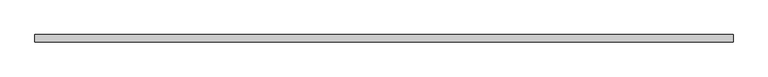
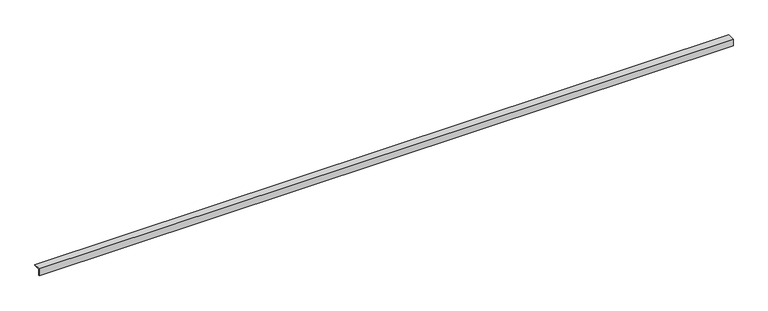
"""IFC4 building model written with IfcOpenShell, lengths in millimetres: proxy geometry, Generic Models 7:Generic Models 1:337419:Generic Models 1:337419 : Generic Models 7:Generic Models 1:337419:15 : Generic Models 7:Generic Models 1:337419:Generic Models 1:337419 : Generic Models 7:Generic Models 1:337419:301336."""

from ifc_helpers import new_model, si_unit, frame, origin, place, context, project, spatial, polyline, outline, extrude, source, transform, mapped, element, save


def generic_models_9543ae2d(model_context):
    return source(origin(), model_context, "Body", "SweptSolid", [
        extrude(outline(polyline([(-536554.1163358, 8576.3695313), (-536503.3163358, 8576.3695313), (-536503.3163358, 8571.6070313), (-536549.3538358, 8571.6070313), (-536549.3538358, 8525.5695312), (-536554.1163358, 8525.5695312), (-536554.1163358, 8576.3695313)])), frame((591306.0367242, 0.0, 0.0), z_axis=(1.0, 0.0, 0.0), x_axis=(0.0, 1.0, 0.0)), (0.0, 0.0, 1.0), 4876.8),
    ])


if __name__ == "__main__":
    model = new_model("IFC4")
    model_context = context("Model", 3, world=origin())
    ifc_project = project(units=[si_unit("LENGTHUNIT", "METRE", prefix="MILLI")], contexts=[model_context])
    site = spatial("IfcSite", under=ifc_project)
    building = spatial("IfcBuilding", under=site)
    placement = place(None, origin())
    generic_models_shape = generic_models_9543ae2d(model_context)
    element("IfcBuildingElementProxy", 1, Name="Generic Models 7:Generic Models 1:337419:Generic Models 1:337419 : Generic Models 7:Generic Models 1:337419:15 : Generic Models 7:Generic Models 1:337419:Generic Models 1:337419 : Generic Models 7:Generic Models 1:337419:301336", ObjectType="Generic Models 7:Generic Models 1:337419:Generic Models 1:337419 : Generic Models 7:Generic Models 1:337419:15 : Generic Models 7:Generic Models 1:337419:Generic Models 1:337419 : Generic Models 7:Generic Models 1:337419:301336", at=placement, inside=building, context=model_context, shape_type="MappedRepresentation", body=[
        mapped(generic_models_shape, transform((0.0, 0.0, 0.0), x_axis=(1.0, 0.0, 0.0), y_axis=(0.0, 1.0, 0.0), z_axis=(0.0, 0.0, 1.0))),
    ])
    save(model, "model.ifc")

# Revit data of these elements
# Type "Generic Models 7:Generic Models 1:337419:Generic Models 1:337419 : Generic Models 7:Generic Models 1:337419:15 : Generic Models 7:Generic Models 1:337419:Generic Models 1:337419 : Generic Models 7:Generic Models 1:337419:301336"
#   NameOverride = "Generic Models 7:Generic Models 1:337419:Generic Models 1:337419 : Generic Models 7:Generic Models 1:337419:301336"
#   ObjectTypeOverride = "Generic Models 1:337419 : Generic Models 7:Generic Models 1:337419"
#   Reference = "Generic Models 1"
#   Tag = "301336"
# Element 1 (IfcBuildingElementProxy, "Generic Models 7:Generic Models 1:337419:Generic Models 1:337419 : Generic Models 7:Generic Models 1:337419:15 : Generic Models 7:Generic Models 1:337419:Generic Models 1:337419 : Generic Models 7:Generic Models 1:337419:301336")
#   Materials on its faces: "GALVANIZED STEEL ANGLE (L2x2x1/4) WITH #12 GRADE 5 SCREWS @ 24\" O.C."
# Materials
#   "GALVANIZED STEEL ANGLE (L2x2x1/4) WITH #12 GRADE 5 SCREWS @ 24\" O.C.": class "Unassigned", colour RGB 210 209 208, transparency 0, Keynote = "M05121300.02", Cost = 0
